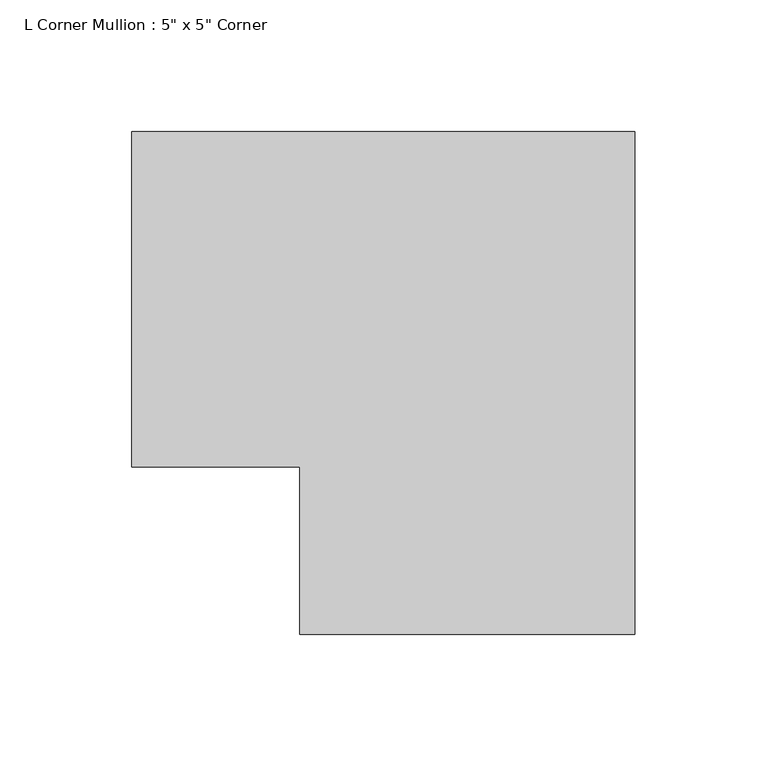
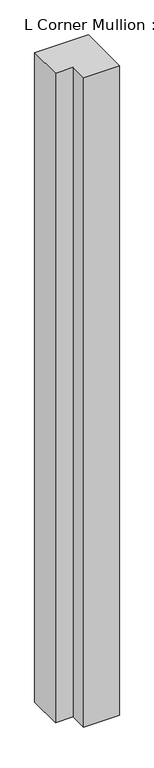
"""IFC4 building model written with IfcOpenShell, lengths in millimetres: member geometry."""

from ifc_helpers import new_model, si_unit, frame, origin, place, context, project, spatial, polyline, outline, extrude, source, transform, mapped, element, save


def member_47e31e63(model_context):
    return source(origin(), model_context, "Body", "SweptSolid", [
        extrude(outline(polyline([(-63.5, -127.0), (-63.5, -63.5), (-127.0, -63.5), (-127.0, 63.5), (63.5, 63.5), (63.5, -127.0), (-63.5, -127.0)])), frame((0.0, 0.0, -2438.4), z_axis=(0.0, 0.0, 1.0), x_axis=(1.0, 0.0, 0.0)), (0.0, 0.0, 1.0), 2438.4),
    ])


if __name__ == "__main__":
    model = new_model("IFC4")
    model_context = context("Model", 3, world=origin())
    ifc_project = project(units=[si_unit("LENGTHUNIT", "METRE", prefix="MILLI")], contexts=[model_context])
    site = spatial("IfcSite", under=ifc_project)
    building = spatial("IfcBuilding", under=site)
    placement = place(None, origin())
    member_shape = member_47e31e63(model_context)
    element("IfcMember", 1, ObjectType="L Corner Mullion : 5\" x 5\" Corner", at=placement, inside=building, context=model_context, shape_type="MappedRepresentation", body=[
        mapped(member_shape, transform((0.0, 0.0, 0.0), x_axis=(1.0, 0.0, 0.0), y_axis=(0.0, 1.0, 0.0), z_axis=(0.0, 0.0, 1.0))),
    ])
    save(model, "model.ifc")

# Revit data of these elements
# Type "L Corner Mullion : 5\" x 5\" Corner"
#   built-in parameter 1007355 = 0.416667 (stored number, unit not read)
#   built-in parameter 1007354 = 0.416667 (stored number, unit not read)
#   built-in parameter 1007304 = 0.416667 (stored number, unit not read)
# Element 1 (IfcMember, "L Corner Mullion : 5\" x 5\" Corner")
#   Materials on its faces: "Metal - Aluminum"
# Materials
#   "Metal - Aluminum": class "Metal", colour RGB 140 140 140, transparency 0
